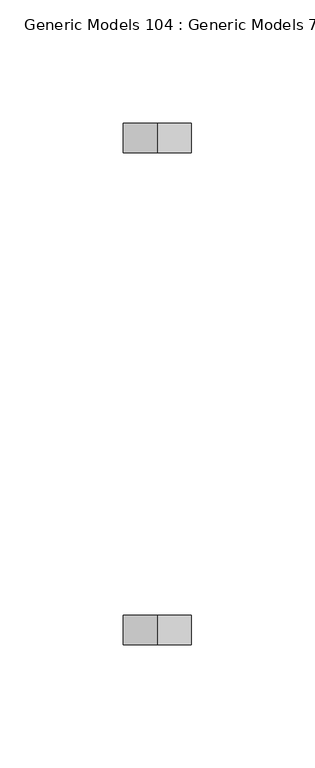
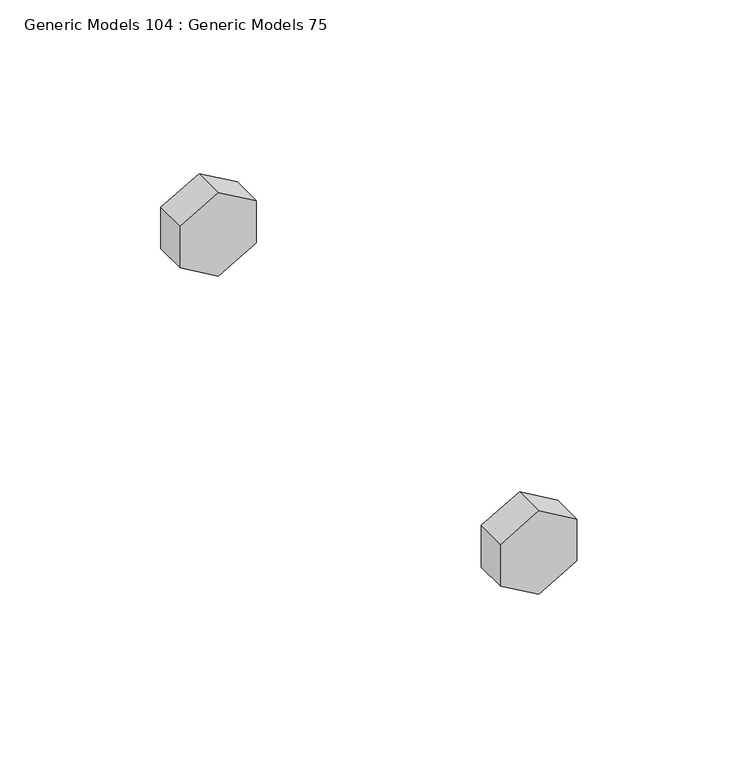
"""IFC4 building model written with IfcOpenShell, lengths in millimetres: proxy geometry, Generic Models 104 : Generic Models 75."""

from ifc_helpers import new_model, si_unit, frame, origin, place, context, project, spatial, polyline, outline, extrude, source, transform, mapped, element, save


def generic_models_104_generic_models_75_e3270acc(model_context):
    return source(origin(), model_context, "Body", "SweptSolid", [
        extrude(outline(polyline([(268917.5462802, 31974.4067029), (268901.7097067, 31974.4067029), (268893.79142, 31988.1215778), (268901.7097067, 32001.8364528), (268917.5462802, 32001.8364528), (268925.464567, 31988.1215778), (268917.5462802, 31974.4067029)])), frame((0.0, 36501.0832942, 0.0), z_axis=(0.0, 1.0, 0.0), x_axis=(0.0, 0.0, 1.0)), (0.0, 0.0, 1.0), 11.90625),
        extrude(outline(polyline([(268917.5462802, 31974.4067029), (268901.7097067, 31974.4067029), (268893.79142, 31988.1215778), (268901.7097067, 32001.8364528), (268917.5462802, 32001.8364528), (268925.464567, 31988.1215778), (268917.5462802, 31974.4067029)])), frame((0.0, 36301.8520442, 0.0), z_axis=(0.0, 1.0, 0.0), x_axis=(0.0, 0.0, 1.0)), (0.0, 0.0, 1.0), 11.90625),
    ])


if __name__ == "__main__":
    model = new_model("IFC4")
    model_context = context("Model", 3, world=origin())
    ifc_project = project(units=[si_unit("LENGTHUNIT", "METRE", prefix="MILLI")], contexts=[model_context])
    site = spatial("IfcSite", under=ifc_project)
    building = spatial("IfcBuilding", under=site)
    placement = place(None, origin())
    generic_models_104_generic_models_75_shape = generic_models_104_generic_models_75_e3270acc(model_context)
    element("IfcBuildingElementProxy", 1, Name="Generic Models 104 : Generic Models 75", ObjectType="Generic Models 104 : Generic Models 75", at=placement, inside=building, context=model_context, shape_type="MappedRepresentation", body=[
        mapped(generic_models_104_generic_models_75_shape, transform((0.0, 0.0, 0.0), x_axis=(1.0, 0.0, 0.0), y_axis=(0.0, 1.0, 0.0), z_axis=(0.0, 0.0, 1.0))),
    ])
    save(model, "model.ifc")

# Revit data of these elements
# Element 1 (IfcBuildingElementProxy, "Generic Models 104 : Generic Models 75")
#   Materials on its faces: "3/4\" GALV. THRU BOLTS"
# Materials
#   "3/4\" GALV. THRU BOLTS": class "Generic", colour RGB 105 69 171, transparency 0, Cost = 0
